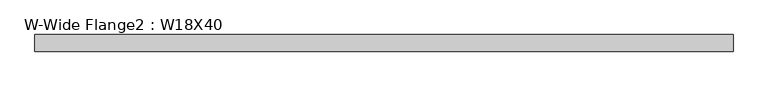
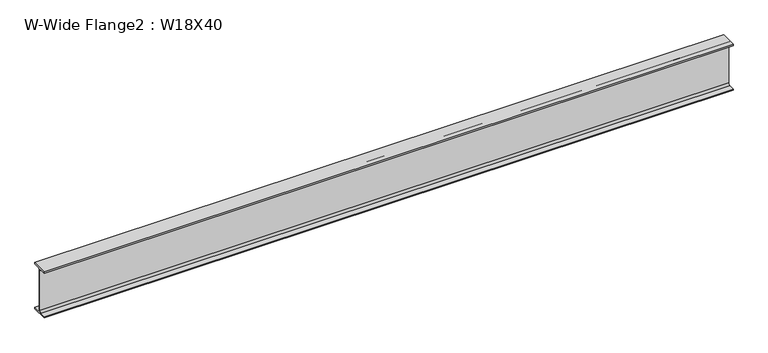
"""IFC4 building model written with IfcOpenShell, lengths in millimetres: beam geometry, W-Wide Flange2 : W18X40."""

from ifc_helpers import new_model, si_unit, point, frame, frame_2d, origin, place, context, project, spatial, polyline, circle_curve, trimmed, segment, composite_curve, outline, extrude, source, transform, mapped, element, save


def w_wide_flange2_w18x40_11743c99(model_context):
    return source(origin(), model_context, "Body", "SweptSolid", [
        extrude(outline(composite_curve([segment(polyline([(76.454, -213.995), (76.454, -227.33), (-76.454, -227.33), (-76.454, -213.995), (-20.828, -213.995)]), True, "CONTINUOUS"), segment(trimmed(circle_curve(frame_2d((-20.828, -197.1675)), 16.8275), [point((-20.828, -213.995))], [point((-4.0005, -197.1675))], True, "CARTESIAN"), True, "CONTINUOUS"), segment(polyline([(-4.0005, -197.1675), (-4.0005, 197.1675)]), True, "CONTINUOUS"), segment(trimmed(circle_curve(frame_2d((-20.828, 197.1675)), 16.8275), [point((-4.0005, 197.1675))], [point((-20.828, 213.995))], True, "CARTESIAN"), True, "CONTINUOUS"), segment(polyline([(-20.828, 213.995), (-76.454, 213.995), (-76.454, 227.33), (76.454, 227.33), (76.454, 213.995), (20.828, 213.995)]), True, "CONTINUOUS"), segment(trimmed(circle_curve(frame_2d((20.828, 197.1675)), 16.8275), [point((20.828, 213.995))], [point((4.0005, 197.1675))], True, "CARTESIAN"), True, "CONTINUOUS"), segment(polyline([(4.0005, 197.1675), (4.0005, -197.1675)]), True, "CONTINUOUS"), segment(trimmed(circle_curve(frame_2d((20.828, -197.1675)), 16.8275), [point((4.0005, -197.1675))], [point((20.828, -213.995))], True, "CARTESIAN"), True, "CONTINUOUS"), segment(polyline([(20.828, -213.995), (76.454, -213.995)]), True, "CONTINUOUS")], self_intersect=False)), frame((-3211.5125, 0.0, 0.0), z_axis=(1.0, 0.0, 0.0), x_axis=(0.0, 1.0, 0.0)), (0.0, 0.0, 1.0), 6423.025),
    ])


if __name__ == "__main__":
    model = new_model("IFC4")
    model_context = context("Model", 3, world=origin())
    ifc_project = project(units=[si_unit("LENGTHUNIT", "METRE", prefix="MILLI")], contexts=[model_context])
    site = spatial("IfcSite", under=ifc_project)
    building = spatial("IfcBuilding", under=site)
    placement = place(None, origin())
    w_wide_flange2_w18x40_shape = w_wide_flange2_w18x40_11743c99(model_context)
    element("IfcBeam", 1, ObjectType="W-Wide Flange2 : W18X40", at=placement, inside=building, context=model_context, shape_type="MappedRepresentation", body=[
        mapped(w_wide_flange2_w18x40_shape, transform((0.0, 0.0, 0.0), x_axis=(1.0, 0.0, 0.0), y_axis=(0.0, 1.0, 0.0), z_axis=(0.0, 0.0, 1.0))),
    ])
    save(model, "model.ifc")

# Revit data of these elements
# Type "W-Wide Flange2 : W18X40"
#   Assembly Code = "B10"
#   W = 40
#   Length [instance default] = 5' - 0"
#   bf = 0' - 6.02"
#   d = 1' - 5.9"
#   k = 0' - 1 3/16"
#   k2 = 0' - 0.6625"
#   tf = 0' - 0.525"
#   tw = 0' - 0.315"
#   A = 0.0819444 SF
#   Structural Material [instance default] = Steel ASTM A992
# Element 1 (IfcBeam, "W-Wide Flange2 : W18X40")
#   Materials on its faces: "Steel ASTM A992"
# Materials
#   "Steel ASTM A992": class "Metal", colour RGB 199 199 199, transparency 0, Description = "Structural steel 50ksi", Cost = 0
